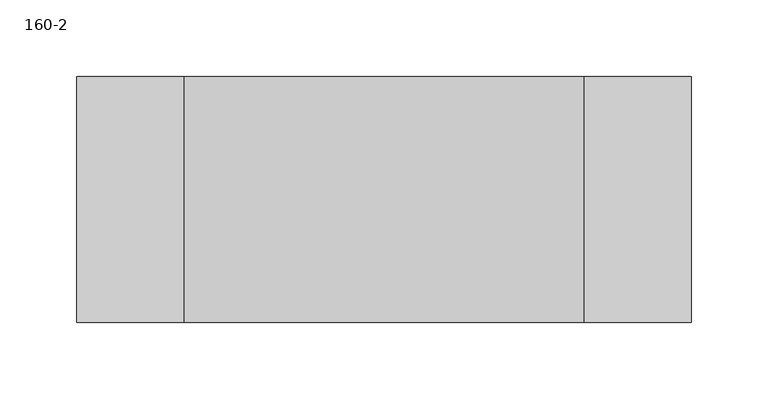
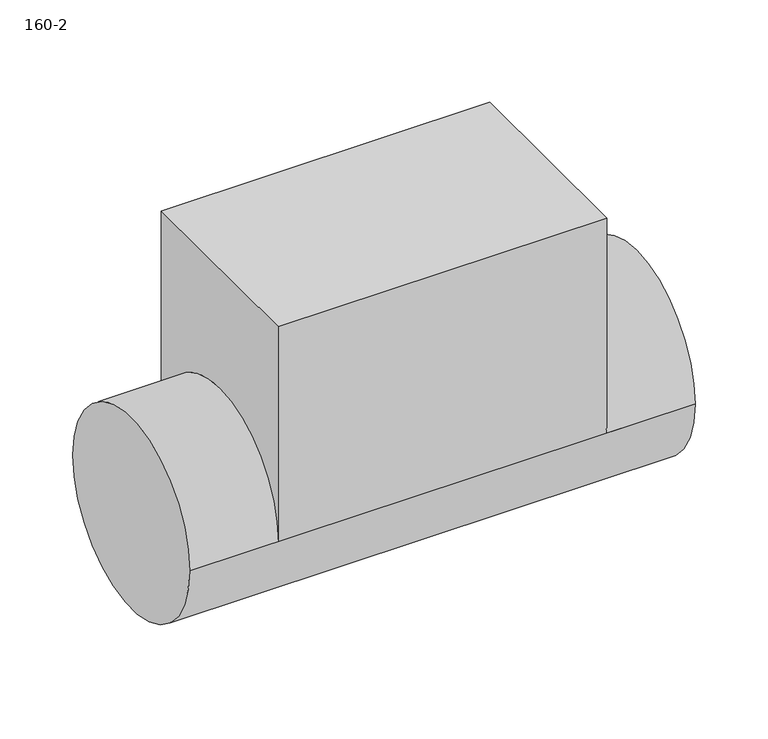
"""IFC4 building model written with IfcOpenShell, lengths in millimetres: proxy geometry, НАГРЕВАТЕЛЬ ЭЛЕКТРИЧЕСКИЙ VKHR-E : 160-2."""

from ifc_helpers import new_model, si_unit, frame, origin, place, context, project, spatial, circle_curve, source, transform, mapped, element, save
from ifc_brep_helpers import plane_surface, cylinder_surface, advanced_brep


def proxy_160_2_af655024(model_context):
    return source(origin(), model_context, "Body", "AdvancedBrep", [
        advanced_brep(
        [(400.0, -80.0, 0.0), (400.0, 80.0, 0.0), (0.0, -80.0, 0.0), (0.0, 80.0, 0.0), (330.0, -80.0, 0.0), (70.0, -80.0, 0.0), (70.0, 80.0, 0.0), (330.0, 80.0, 0.0), (330.0, 80.0, 180.0), (70.0, 80.0, 180.0), (70.0, -80.0, 180.0), (330.0, -80.0, 180.0)],
        [
            (0, 1, circle_curve(frame((400.0, 0.0, 0.0), z_axis=(1.0, 0.0, 0.0), x_axis=(0.0, 1.0, 0.0)), 80.0)),
            (1, 0, circle_curve(frame((400.0, 0.0, 0.0), z_axis=(1.0, 0.0, 0.0), x_axis=(0.0, 1.0, 0.0)), 80.0)),
            (2, 3, circle_curve(frame((0.0, 0.0, 0.0), z_axis=(-1.0, 0.0, 0.0), x_axis=(0.0, 1.0, 0.0)), 80.0)),
            (3, 2, circle_curve(frame((0.0, 0.0, 0.0), z_axis=(-1.0, 0.0, 0.0), x_axis=(0.0, 1.0, 0.0)), 80.0)),
            (0, 4),
            (4, 5),
            (5, 2),
            (3, 6),
            (6, 7),
            (7, 1),
            (7, 4, circle_curve(frame((330.0, 0.0, 0.0), z_axis=(1.0, 0.0, 0.0), x_axis=(0.0, 1.0, 0.0)), 80.0)),
            (5, 6, circle_curve(frame((70.0, 0.0, 0.0), z_axis=(-1.0, 0.0, 0.0), x_axis=(0.0, 1.0, 0.0)), 80.0)),
            (8, 9),
            (9, 10),
            (10, 11),
            (11, 8),
            (8, 7),
            (6, 9),
            (5, 10),
            (4, 11),
        ],
        [
            plane_surface(frame((400.0, 80.0, 0.0), z_axis=(1.0, 0.0, 0.0), x_axis=(0.0, 0.0, 1.0))),
            plane_surface(frame((0.0, 80.0, 0.0), z_axis=(-1.0, 0.0, 0.0), x_axis=(0.0, 0.0, -1.0))),
            cylinder_surface(frame((0.0, 0.0, 0.0), z_axis=(1.0, 0.0, 0.0), x_axis=(0.0, 1.0, 0.0)), 80.0),
            plane_surface(frame((70.0, 80.0, 180.0), z_axis=(0.0, 0.0, 1.0), x_axis=(-1.0, 0.0, 0.0))),
            plane_surface(frame((330.0, 80.0, 180.0), z_axis=(0.0, 1.0, 0.0), x_axis=(0.0, 0.0, -1.0))),
            plane_surface(frame((70.0, 80.0, 180.0), z_axis=(-1.0, 0.0, 0.0), x_axis=(0.0, 0.0, -1.0))),
            plane_surface(frame((70.0, -80.0, 180.0), z_axis=(0.0, -1.0, 0.0), x_axis=(0.0, 0.0, -1.0))),
            plane_surface(frame((330.0, -80.0, 180.0), z_axis=(1.0, 0.0, 0.0), x_axis=(0.0, 0.0, -1.0))),
        ],
        [
            (0, [[1, 2]]),
            (1, [[3, 4]]),
            (2, [[-1, 5, 6, 7, -4, 8, 9, 10]]),
            (2, [[-2, -10, 11, -5]]),
            (2, [[-3, -7, 12, -8]]),
            (3, [[13, 14, 15, 16]]),
            (4, [[-13, 17, -9, 18]]),
            (5, [[-14, -18, -12, 19]]),
            (6, [[-15, -19, -6, 20]]),
            (7, [[-16, -20, -11, -17]]),
        ],
    ),
    ])


if __name__ == "__main__":
    model = new_model("IFC4")
    model_context = context("Model", 3, world=origin())
    ifc_project = project(units=[si_unit("LENGTHUNIT", "METRE", prefix="MILLI")], contexts=[model_context])
    site = spatial("IfcSite", under=ifc_project)
    building = spatial("IfcBuilding", under=site)
    placement = place(None, origin())
    proxy_160_2_shape = proxy_160_2_af655024(model_context)
    element("IfcBuildingElementProxy", 1, Name="НАГРЕВАТЕЛЬ ЭЛЕКТРИЧЕСКИЙ VKHR-E : 160-2", ObjectType="НАГРЕВАТЕЛЬ ЭЛЕКТРИЧЕСКИЙ VKHR-E : 160-2", at=placement, inside=building, context=model_context, shape_type="MappedRepresentation", body=[
        mapped(proxy_160_2_shape, transform((0.0, 0.0, 0.0), x_axis=(1.0, 0.0, 0.0), y_axis=(0.0, 1.0, 0.0), z_axis=(0.0, 0.0, 1.0))),
    ])
    save(model, "model.ifc")

# Revit data of these elements
# Type "НАГРЕВАТЕЛЬ ЭЛЕКТРИЧЕСКИЙ VKHR-E : 160-2"
#   ADSK_Наименование = "Нагреватель электрический VKHR-E"
#   ADSK_Марка = "VKHR-E 100/0,5"
#   L = 400 mm
#   H = 180 mm
#   D = 160 mm
#   Default Elevation = 0
